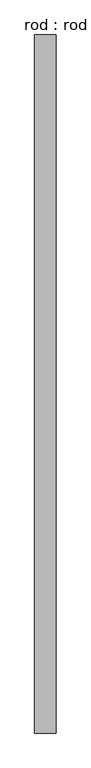
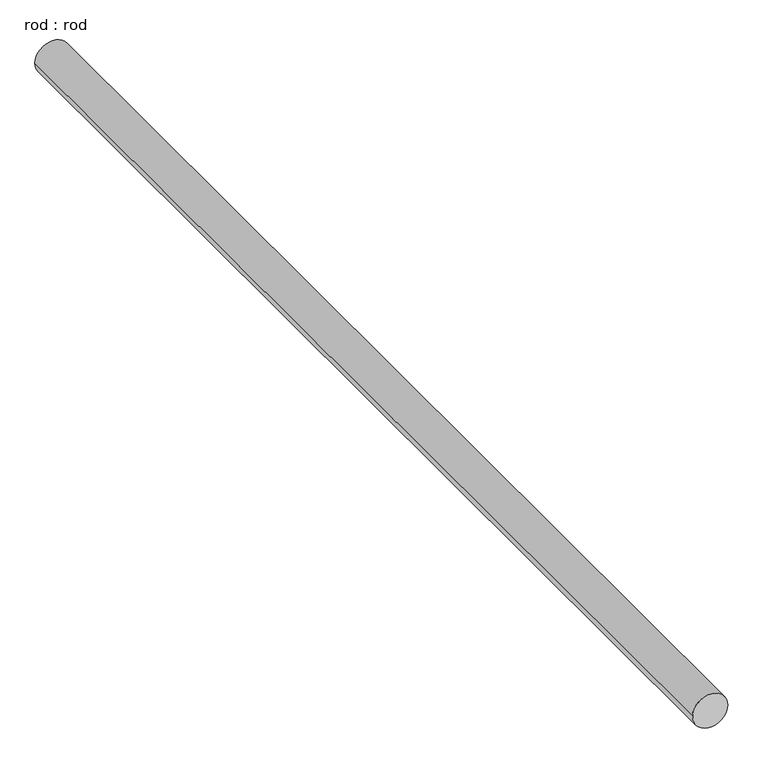
"""IFC4 building model written with IfcOpenShell, lengths in millimetres: proxy geometry, rod : rod."""

from ifc_helpers import new_model, si_unit, point, frame, frame_2d, origin, place, context, project, spatial, circle_curve, trimmed, segment, composite_curve, outline, extrude, source, transform, mapped, element, save


def rod_rod_1726985c(model_context):
    return source(origin(), model_context, "Body", "SweptSolid", [
        extrude(outline(composite_curve([segment(trimmed(circle_curve(frame_2d((0.0108462, 0.0)), 200.0), [point((0.0108462, 200.0))], [point((0.0108462, -200.0))], False, "CARTESIAN"), True, "CONTINUOUS"), segment(trimmed(circle_curve(frame_2d((0.0108462, 0.0)), 200.0), [point((0.0108462, -200.0))], [point((0.0108462, 200.0))], False, "CARTESIAN"), True, "CONTINUOUS")], self_intersect=False)), frame((0.0, -2391.0986057, 0.0), z_axis=(0.0, 1.0, 0.0), x_axis=(0.0, 0.0, 1.0)), (0.0, 0.0, 1.0), 12967.654442),
    ])


if __name__ == "__main__":
    model = new_model("IFC4")
    model_context = context("Model", 3, world=origin())
    ifc_project = project(units=[si_unit("LENGTHUNIT", "METRE", prefix="MILLI")], contexts=[model_context])
    site = spatial("IfcSite", under=ifc_project)
    building = spatial("IfcBuilding", under=site)
    placement = place(None, origin())
    rod_rod_shape = rod_rod_1726985c(model_context)
    element("IfcBuildingElementProxy", 1, Name="rod : rod", ObjectType="rod : rod", at=placement, inside=building, context=model_context, shape_type="MappedRepresentation", body=[
        mapped(rod_rod_shape, transform((0.0, 0.0, 0.0), x_axis=(1.0, 0.0, 0.0), y_axis=(0.0, 1.0, 0.0), z_axis=(0.0, 0.0, 1.0))),
    ])
    save(model, "model.ifc")

# Revit data of these elements
# Type "rod : rod"
#   Default Elevation = 0
